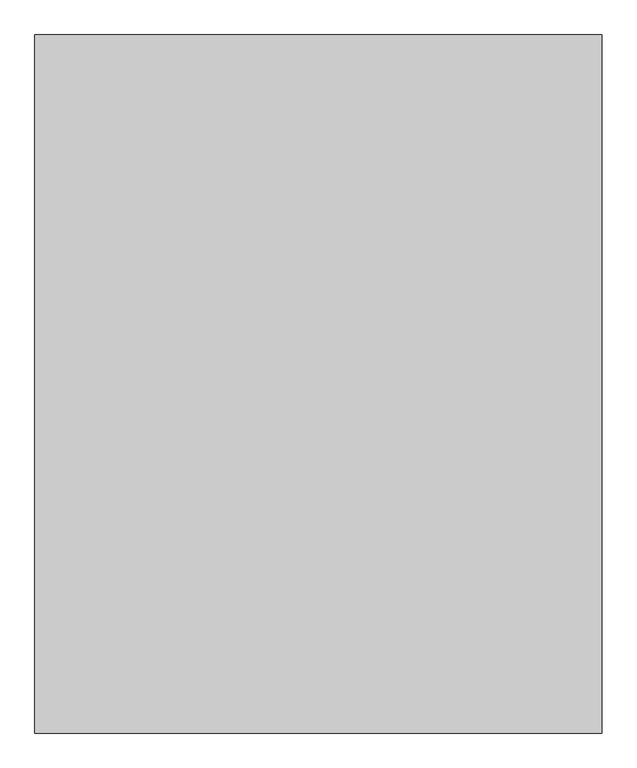
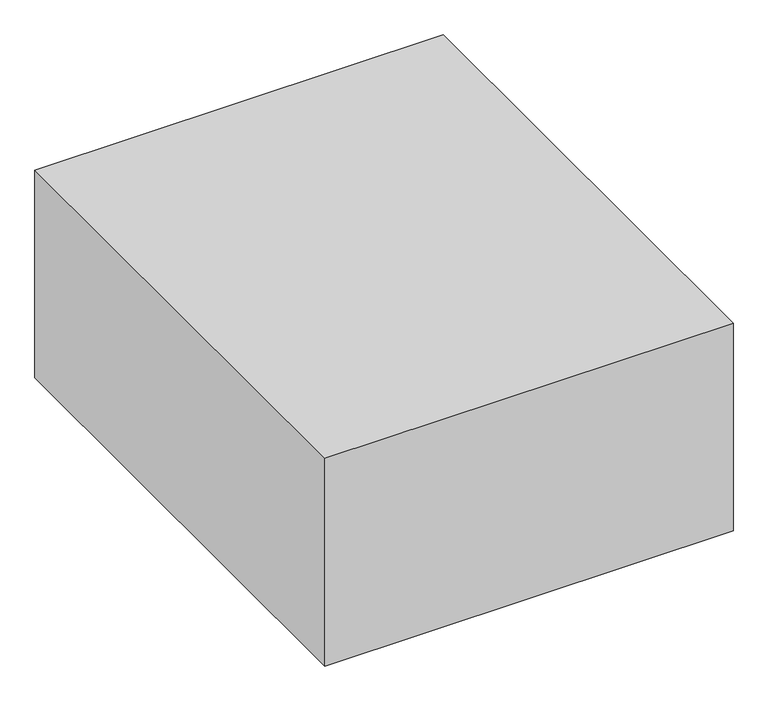
"""IFC4 building model written with IfcOpenShell, lengths in millimetres: proxy geometry, Space Planning Box_hec : Space Planning Box_hec."""

from ifc_helpers import new_model, si_unit, origin, origin_with_axes, place, context, project, spatial, polyline, outline, extrude, source, transform, mapped, element, save


def generic_models_70f6ae48(model_context):
    return source(origin(), model_context, "Body", "SweptSolid", [
        extrude(outline(polyline([(3250.0, 4000.0), (3250.0, -4000.0), (-3250.0, -4000.0), (-3250.0, 4000.0), (3250.0, 4000.0)])), origin_with_axes(), (0.0, 0.0, 1.0), 3500.0),
    ])


if __name__ == "__main__":
    model = new_model("IFC4")
    model_context = context("Model", 3, world=origin())
    ifc_project = project(units=[si_unit("LENGTHUNIT", "METRE", prefix="MILLI")], contexts=[model_context])
    site = spatial("IfcSite", under=ifc_project)
    building = spatial("IfcBuilding", under=site)
    placement = place(None, origin())
    generic_models_shape = generic_models_70f6ae48(model_context)
    element("IfcBuildingElementProxy", 1, Name="Space Planning Box_hec : Space Planning Box_hec", ObjectType="Space Planning Box_hec : Space Planning Box_hec", at=placement, inside=building, context=model_context, shape_type="MappedRepresentation", body=[
        mapped(generic_models_shape, transform((0.0, 0.0, 0.0), x_axis=(1.0, 0.0, 0.0), y_axis=(0.0, 1.0, 0.0), z_axis=(0.0, 0.0, 1.0))),
    ])
    save(model, "model.ifc")

# Revit data of these elements
# Type "Space Planning Box_hec : Space Planning Box_hec"
#   Type Comments = "..."
#   Room Name [instance default] = "?"
#   Interior Finish [instance default] = ""
#   Exterior Finish [instance default] = ""
#   Department [instance default] = ""
#   Assembly Code = "..."
#   ceiling height [instance default] = 0
#   Width [instance default] = 1524 mm
#   Program Area [instance default] = 0.00 m²
#   Length [instance default] = 1524 mm
#   Height [instance default] = 1524 mm
#   Area [instance default] = 2.32258 m²
#   Fill Color [instance default] = Cyan
#   Default Elevation = 0
# Element 1 (IfcBuildingElementProxy, "Space Planning Box_hec : Space Planning Box_hec")
#   Room Name = "Meeting Room-2"
#   Exterior Finish = "RF1..N/A,,EW1..N/A..N/A"
#   Department = "AR"
#   Width = 6500 mm
#   Program Area = 52.00 m²
#   Length = 8000 mm
#   Height = 3500 mm
#   Area = 52.00 m²
#   Materials on its faces: "Cyan"
# Materials
#   "Cyan": class "Generic", colour RGB 0 255 255, transparency 0.2, Cost = 0
